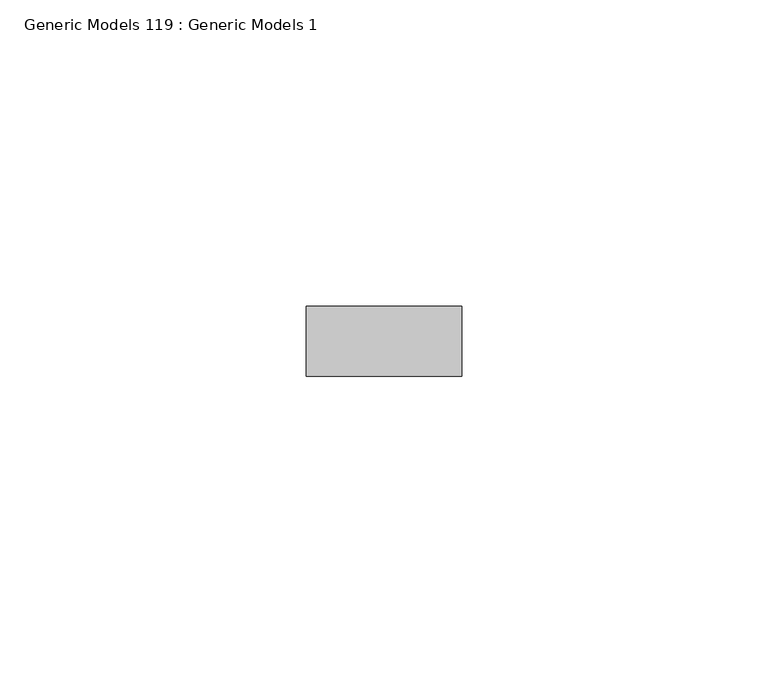
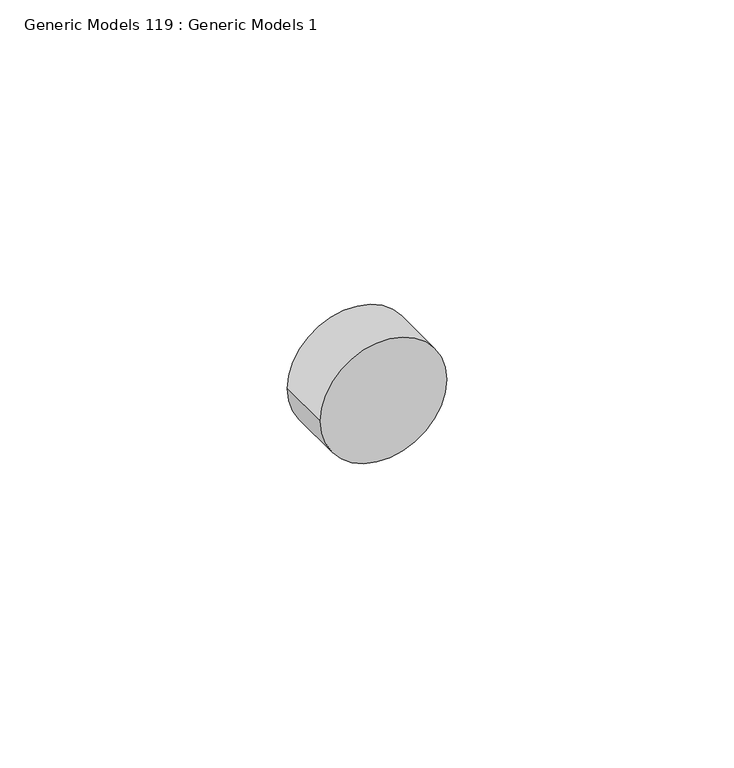
"""IFC4 building model written with IfcOpenShell, lengths in millimetres: proxy geometry, Generic Models 119 : Generic Models 1."""

from ifc_helpers import new_model, si_unit, point, frame, frame_2d, origin, place, context, project, spatial, circle_curve, trimmed, segment, composite_curve, outline, extrude, source, transform, mapped, element, save


def generic_models_119_generic_models_1_3803042c(model_context):
    return source(origin(), model_context, "Body", "SweptSolid", [
        extrude(outline(composite_curve([segment(trimmed(circle_curve(frame_2d((38031.9291136, 7018.1346014)), 12.7), [point((38031.9291136, 7030.8346014))], [point((38031.9291136, 7005.4346014))], False, "CARTESIAN"), True, "CONTINUOUS"), segment(trimmed(circle_curve(frame_2d((38031.9291136, 7018.1346014)), 12.7), [point((38031.9291136, 7005.4346014))], [point((38031.9291136, 7030.8346014))], False, "CARTESIAN"), True, "CONTINUOUS")], self_intersect=False)), frame((0.0, 1836.9202358, 0.0), z_axis=(0.0, 1.0, 0.0), x_axis=(0.0, 0.0, 1.0)), (0.0, 0.0, 1.0), 11.4464372),
    ])


if __name__ == "__main__":
    model = new_model("IFC4")
    model_context = context("Model", 3, world=origin())
    ifc_project = project(units=[si_unit("LENGTHUNIT", "METRE", prefix="MILLI")], contexts=[model_context])
    site = spatial("IfcSite", under=ifc_project)
    building = spatial("IfcBuilding", under=site)
    placement = place(None, origin())
    generic_models_119_generic_models_1_shape = generic_models_119_generic_models_1_3803042c(model_context)
    element("IfcBuildingElementProxy", 1, Name="Generic Models 119 : Generic Models 1", ObjectType="Generic Models 119 : Generic Models 1", at=placement, inside=building, context=model_context, shape_type="MappedRepresentation", body=[
        mapped(generic_models_119_generic_models_1_shape, transform((0.0, 0.0, 0.0), x_axis=(1.0, 0.0, 0.0), y_axis=(0.0, 1.0, 0.0), z_axis=(0.0, 0.0, 1.0))),
    ])
    save(model, "model.ifc")

# Revit data of these elements
# Element 1 (IfcBuildingElementProxy, "Generic Models 119 : Generic Models 1")
#   Materials on its faces: "S.S. LAG BOLT - SEE STRUCT. DWGS"
# Materials
#   "S.S. LAG BOLT - SEE STRUCT. DWGS": class "Generic", colour RGB 120 120 120, transparency 0, Cost = 0
